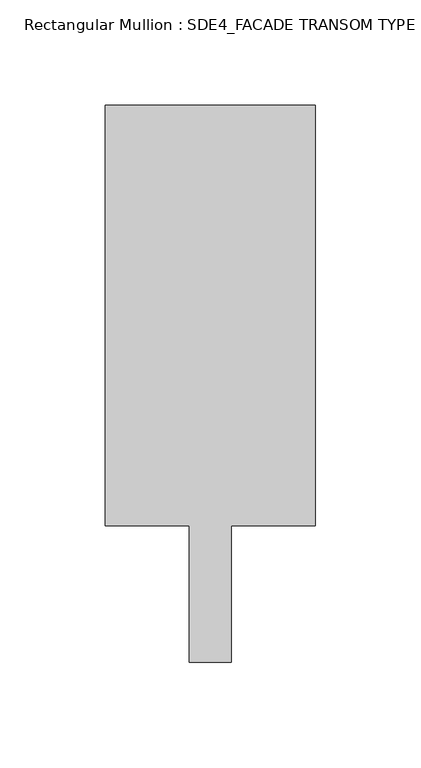
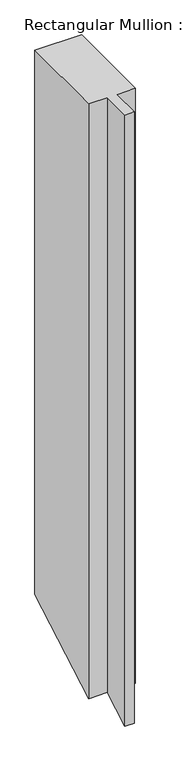
"""IFC4 building model written with IfcOpenShell, lengths in millimetres: member geometry, Rectangular Mullion : SDE4_FACADE TRANSOM TYPE 2."""

from ifc_helpers import new_model, si_unit, origin, place, context, project, spatial, faceted_brep, source, transform, mapped, element, save


def rectangular_mullion_sde4_facade_transom_type_2_487c5f16(model_context):
    return source(origin(), model_context, "Body", "Brep", [
        faceted_brep([(50.0, 132.5, 0.0), (-50.0, 132.5, 0.0), (-50.0, -67.5, 0.0), (-10.0, -67.5, 0.0), (-10.0, -132.5, 0.0), (10.0, -132.5, 0.0), (10.0, -67.5, 0.0), (50.0, -67.5, 0.0), (50.0, 132.5, -1234.1646793), (-50.0, 132.5, -1234.1646793), (-50.0, -67.5, -1349.5399841), (-10.0, -67.5, -1349.5399841), (-10.0, -132.5, -1387.0369581), (10.0, -132.5, -1387.0369581), (10.0, -67.5, -1349.5399841), (50.0, -67.5, -1349.5399841)], [[[0, 1, 2, 3, 4, 5, 6, 7]], [[1, 0, 8, 9]], [[2, 1, 9, 10]], [[3, 2, 10, 11]], [[4, 3, 11, 12]], [[5, 4, 12, 13]], [[6, 5, 13, 14]], [[7, 6, 14, 15]], [[0, 7, 15, 8]], [[8, 15, 14, 13, 12, 11, 10, 9]]]),
    ])


if __name__ == "__main__":
    model = new_model("IFC4")
    model_context = context("Model", 3, world=origin())
    ifc_project = project(units=[si_unit("LENGTHUNIT", "METRE", prefix="MILLI")], contexts=[model_context])
    site = spatial("IfcSite", under=ifc_project)
    building = spatial("IfcBuilding", under=site)
    placement = place(None, origin())
    rectangular_mullion_sde4_facade_transom_type_2_shape = rectangular_mullion_sde4_facade_transom_type_2_487c5f16(model_context)
    element("IfcMember", 1, ObjectType="Rectangular Mullion : SDE4_FACADE TRANSOM TYPE 2", at=placement, inside=building, context=model_context, shape_type="MappedRepresentation", body=[
        mapped(rectangular_mullion_sde4_facade_transom_type_2_shape, transform((0.0, 0.0, 0.0), x_axis=(1.0, 0.0, 0.0), y_axis=(0.0, 1.0, 0.0), z_axis=(0.0, 0.0, 1.0))),
    ])
    save(model, "model.ifc")

# Revit data of these elements
# Type "Rectangular Mullion : SDE4_FACADE TRANSOM TYPE 2"
#   built-in parameter 1007322 = 0.869423 (stored number, unit not read)
#   built-in parameter 1007321 = 0.164042 (stored number, unit not read)
#   built-in parameter 1007320 = 0.164042 (stored number, unit not read)
